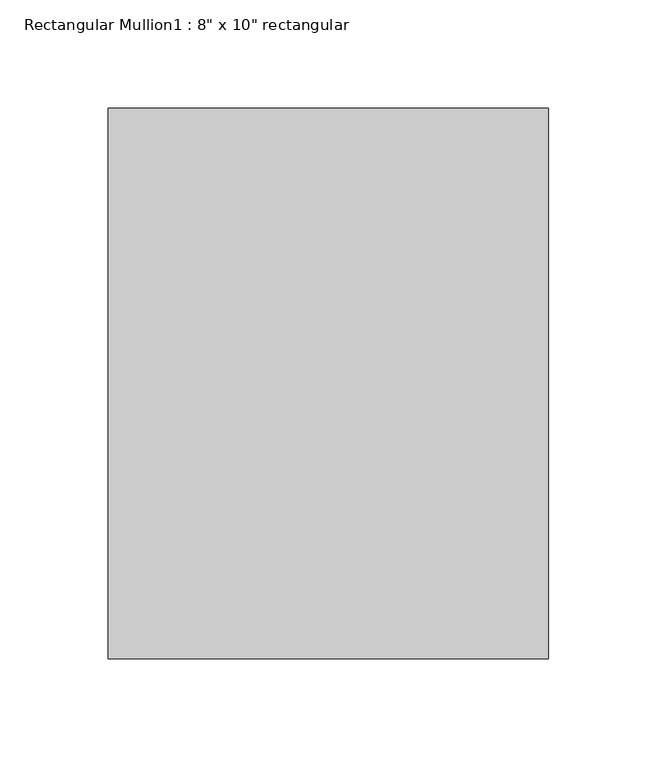
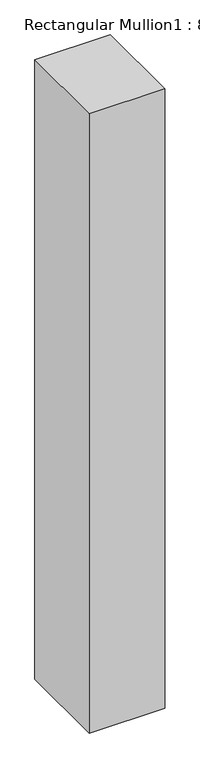
"""IFC4 building model written with IfcOpenShell, lengths in millimetres: member geometry."""

import ifcopenshell
import ifcopenshell.guid

model = None  # the IFC model being written
_history = None  # IfcOwnerHistory: only IFC2X3 demands one
_inside = {}  # id of a spatial element -> (the spatial element, [elements in it])
_under = {}  # id of a project, library or spatial element -> (it, [spatial elements below it])
_declared = {}  # id of a project -> (the project, [libraries it declares])
_typed = {}  # id of a type object -> (the type object, [elements of that type])
_made_of = {}  # id of a material, layer set ... -> (it, [elements and type objects made of it])


def new_model(schema):
    """Start an empty IFC model of exactly this schema.

    Asked for "IFC4X3", IfcOpenShell would pick the latest addendum, in which some entities
    have other attributes; the version numbers below select the first issue.
    IFC2X3 requires an IfcOwnerHistory on every rooted entity: one is made here for all.
    """
    global model, _history
    if schema == "IFC4X3":
        model = ifcopenshell.file(schema_version=(4, 3, 0, 0))
    else:
        model = ifcopenshell.file(schema=schema)
    _inside.clear()
    _under.clear()
    _declared.clear()
    _typed.clear()
    _made_of.clear()
    _history = None
    if model.schema == "IFC2X3":
        org = make("IfcOrganization", Name="unknown")
        user = make(
            "IfcPersonAndOrganization",
            ThePerson=make("IfcPerson", FamilyName="unknown"),
            TheOrganization=org,
        )
        app = make(
            "IfcApplication",
            ApplicationDeveloper=org,
            Version="unknown",
            ApplicationFullName="unknown",
            ApplicationIdentifier="unknown",
        )
        _history = make(
            "IfcOwnerHistory",
            OwningUser=user,
            OwningApplication=app,
            ChangeAction="ADDED",
            CreationDate=0,
        )
    return model


def make(cls, **values):
    """One entity of the class cls with the attributes given. An attribute that is None is left unset."""
    return model.create_entity(
        cls, **{name: value for name, value in values.items() if value is not None}
    )


def rooted(cls, **values):
    """An entity with a GlobalId (a new one), such as an element, a storey or a relation."""
    return make(cls, GlobalId=ifcopenshell.guid.new(), OwnerHistory=_history, **values)


def si_unit(unit_type, name, prefix=None):
    """IfcSIUnit, for example si_unit("LENGTHUNIT", "METRE", prefix="MILLI")."""
    return make("IfcSIUnit", UnitType=unit_type, Prefix=prefix, Name=name)


def assignment(units):
    """IfcUnitAssignment: the units of a project."""
    return None if units is None else make("IfcUnitAssignment", Units=units)


def point(xyz):
    """IfcCartesianPoint."""
    return None if xyz is None else make("IfcCartesianPoint", Coordinates=xyz)


def direction(xyz):
    """IfcDirection."""
    return None if xyz is None else make("IfcDirection", DirectionRatios=xyz)


def frame(location, z_axis=None, x_axis=None):
    """IfcAxis2Placement3D, a coordinate frame: its origin and axes. An axis left out is left unset."""
    return make(
        "IfcAxis2Placement3D",
        Location=point(location),
        Axis=direction(z_axis),
        RefDirection=direction(x_axis),
    )


def origin():
    """The frame at (0, 0, 0) with its axes left unset."""
    return frame((0.0, 0.0, 0.0))


def place(relative_to, where):
    """IfcLocalPlacement: puts the frame where relative to a parent placement (None: the world)."""
    return make(
        "IfcLocalPlacement", PlacementRelTo=relative_to, RelativePlacement=where
    )


def context(
    kind, dimensions, precision=None, world=None, true_north=None, identifier=None
):
    """IfcGeometricRepresentationContext, for example the 3D "Model" context."""
    return make(
        "IfcGeometricRepresentationContext",
        ContextIdentifier=identifier,
        ContextType=kind,
        CoordinateSpaceDimension=dimensions,
        Precision=precision,
        WorldCoordinateSystem=world,
        TrueNorth=true_north,
    )


def project(units=None, contexts=None):
    """IfcProject with its units and contexts."""
    return rooted(
        "IfcProject",
        Name="project",
        RepresentationContexts=contexts,
        UnitsInContext=assignment(units),
    )


def spatial(cls, under=None, at=None, **own):
    """A site, building, storey or space (cls), placed at a placement, below another one or the project."""
    s = rooted(cls, ObjectPlacement=at, **own)
    if under is not None:
        _under.setdefault(under.id(), (under, []))[1].append(s)
    return s


def polyline(points):
    """IfcPolyline through the points."""
    return make("IfcPolyline", Points=[point(p) for p in points])


def outline(outer, holes=None, kind="AREA"):
    """IfcArbitraryClosedProfileDef: a profile drawn as a closed curve; with holes, ...WithVoids."""
    if holes is None:
        return make("IfcArbitraryClosedProfileDef", ProfileType=kind, OuterCurve=outer)
    return make(
        "IfcArbitraryProfileDefWithVoids",
        ProfileType=kind,
        OuterCurve=outer,
        InnerCurves=holes,
    )


def extrude(swept, where, along, depth):
    """IfcExtrudedAreaSolid: the profile swept, set in the frame where, extruded along a direction by depth."""
    return make(
        "IfcExtrudedAreaSolid",
        SweptArea=swept,
        Position=where,
        ExtrudedDirection=direction(along),
        Depth=depth,
    )


def shape(context_of_items, identifier, shape_type, items):
    """IfcShapeRepresentation: the items that make up one representation, for example the "Body"."""
    return make(
        "IfcShapeRepresentation",
        ContextOfItems=context_of_items,
        RepresentationIdentifier=identifier,
        RepresentationType=shape_type,
        Items=items,
    )


def source(mapping_origin, context_of_items, identifier, shape_type, items):
    """IfcRepresentationMap: a shape defined once, which mapped items show again and again."""
    return make(
        "IfcRepresentationMap",
        MappingOrigin=mapping_origin,
        MappedRepresentation=shape(context_of_items, identifier, shape_type, items),
    )


def transform(
    local_origin,
    x_axis=None,
    y_axis=None,
    z_axis=None,
    scale=None,
    scale2=None,
    scale3=None,
    uniform=True,
):
    """IfcCartesianTransformationOperator3D, or its non-uniform kind. x_axis, y_axis, z_axis: its Axis1, 2, 3."""
    if uniform:
        return make(
            "IfcCartesianTransformationOperator3D",
            Axis1=direction(x_axis),
            Axis2=direction(y_axis),
            LocalOrigin=point(local_origin),
            Scale=scale,
            Axis3=direction(z_axis),
        )
    return make(
        "IfcCartesianTransformationOperator3DnonUniform",
        Axis1=direction(x_axis),
        Axis2=direction(y_axis),
        LocalOrigin=point(local_origin),
        Scale=scale,
        Axis3=direction(z_axis),
        Scale2=scale2,
        Scale3=scale3,
    )


def mapped(mapping_source, mapping_target):
    """IfcMappedItem: shows the shape of a source again, moved by a transform."""
    return make(
        "IfcMappedItem", MappingSource=mapping_source, MappingTarget=mapping_target
    )


def made_of(thing, what):
    """Note that an element or type object is made of a material, layer set ...; save() writes the relation."""
    if what is not None:
        _made_of.setdefault(what.id(), (what, []))[1].append(thing)
    return thing


def element(
    cls,
    number,
    at=None,
    inside=None,
    cuts=None,
    type_object=None,
    material=None,
    context=None,
    identifier="Body",
    shape_type=None,
    held_by="IfcProductDefinitionShape",
    body=None,
    shapes=None,
    **own,
):
    """One element of the class cls, such as IfcWall. Its Tag is "e" and its number.

    at: its placement. inside: the storey or other place that contains it. cuts: it is an
    opening in that element (IfcRelVoidsElement). A single representation is given by context,
    identifier, shape_type and body (its items); several are given by shapes. held_by: the class
    of the entity that holds the representations. save() writes the other relations.
    """
    e = rooted(cls, Tag="e%d" % number, ObjectPlacement=at, **own)
    if body is not None:
        shapes = [shape(context, identifier, shape_type, body)]
    if shapes is not None:
        e.Representation = make(held_by, Representations=shapes)
    if inside is not None:
        _inside.setdefault(inside.id(), (inside, []))[1].append(e)
    if cuts is not None:
        rooted(
            "IfcRelVoidsElement", RelatingBuildingElement=cuts, RelatedOpeningElement=e
        )
    if type_object is not None:
        _typed.setdefault(type_object.id(), (type_object, []))[1].append(e)
    return made_of(e, material)


def aggregate(whole, parts):
    """IfcRelAggregates: a whole, such as a stair, and the parts it consists of."""
    return rooted("IfcRelAggregates", RelatingObject=whole, RelatedObjects=parts)


def save(model, path):
    """Write the relations noted so far, then the file.

    IfcRelAggregates (storeys below a building ...), IfcRelContainedInSpatialStructure (elements
    in a storey), IfcRelDefinesByType, IfcRelAssociatesMaterial and IfcRelDeclares: one each for
    every whole, place, type object, material and project.
    """
    for whole, parts in _under.values():
        aggregate(whole, parts)
    for where, things in _inside.values():
        rooted(
            "IfcRelContainedInSpatialStructure",
            RelatedElements=things,
            RelatingStructure=where,
        )
    for kind, things in _typed.values():
        rooted("IfcRelDefinesByType", RelatedObjects=things, RelatingType=kind)
    for what, things in _made_of.values():
        rooted("IfcRelAssociatesMaterial", RelatedObjects=things, RelatingMaterial=what)
    for by, libraries in _declared.values():
        rooted("IfcRelDeclares", RelatingContext=by, RelatedDefinitions=libraries)
    model.write(path)


def member_707c4438(model_context):
    return source(origin(), model_context, "Body", "SweptSolid", [
        extrude(outline(polyline([(101.6, 127.0), (101.6, -127.0), (-101.6, -127.0), (-101.6, 127.0), (101.6, 127.0)])), frame((0.0, 0.0, -1765.3), z_axis=(0.0, 0.0, 1.0), x_axis=(1.0, 0.0, 0.0)), (0.0, 0.0, 1.0), 1765.3),
    ])


if __name__ == "__main__":
    model = new_model("IFC4")
    model_context = context("Model", 3, world=origin())
    ifc_project = project(units=[si_unit("LENGTHUNIT", "METRE", prefix="MILLI")], contexts=[model_context])
    site = spatial("IfcSite", under=ifc_project)
    building = spatial("IfcBuilding", under=site)
    placement = place(None, origin())
    member_shape = member_707c4438(model_context)
    element("IfcMember", 1, ObjectType="Rectangular Mullion1 : 8\" x 10\" rectangular", at=placement, inside=building, context=model_context, shape_type="MappedRepresentation", body=[
        mapped(member_shape, transform((0.0, 0.0, 0.0), x_axis=(1.0, 0.0, 0.0), y_axis=(0.0, 1.0, 0.0), z_axis=(0.0, 0.0, 1.0))),
    ])
    save(model, "model.ifc")

# Revit data of these elements
# Type "Rectangular Mullion1 : 8\" x 10\" rectangular"
#   built-in parameter 1007304 = 0.833333 (stored number, unit not read)
#   built-in parameter 1007301 = 0.333333 (stored number, unit not read)
#   built-in parameter 1007300 = 0.333333 (stored number, unit not read)
# Element 1 (IfcMember, "Rectangular Mullion1 : 8\" x 10\" rectangular")
#   Materials on its faces: "support-frame"
# Materials
#   "support-frame": class "Unassigned", colour RGB 233 233 233, transparency 0, Cost = 0
